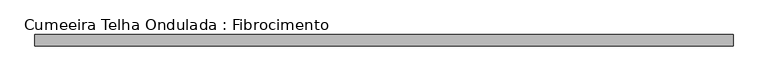
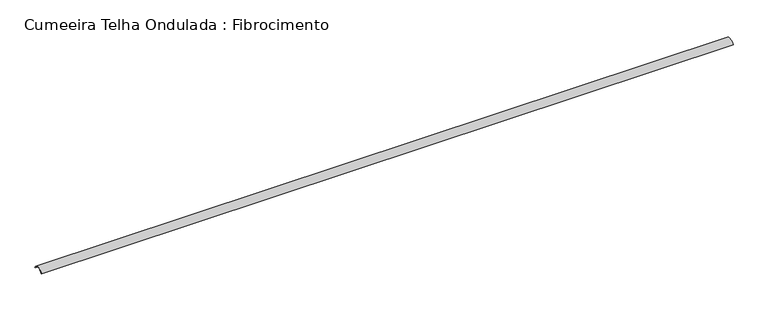
"""IFC4 building model written with IfcOpenShell, lengths in millimetres: beam geometry, Cumeeira Telha Ondulada : Fibrocimento."""

import ifcopenshell
import ifcopenshell.guid

model = None  # the IFC model being written
_history = None  # IfcOwnerHistory: only IFC2X3 demands one
_inside = {}  # id of a spatial element -> (the spatial element, [elements in it])
_under = {}  # id of a project, library or spatial element -> (it, [spatial elements below it])
_declared = {}  # id of a project -> (the project, [libraries it declares])
_typed = {}  # id of a type object -> (the type object, [elements of that type])
_made_of = {}  # id of a material, layer set ... -> (it, [elements and type objects made of it])


def new_model(schema):
    """Start an empty IFC model of exactly this schema.

    Asked for "IFC4X3", IfcOpenShell would pick the latest addendum, in which some entities
    have other attributes; the version numbers below select the first issue.
    IFC2X3 requires an IfcOwnerHistory on every rooted entity: one is made here for all.
    """
    global model, _history
    if schema == "IFC4X3":
        model = ifcopenshell.file(schema_version=(4, 3, 0, 0))
    else:
        model = ifcopenshell.file(schema=schema)
    _inside.clear()
    _under.clear()
    _declared.clear()
    _typed.clear()
    _made_of.clear()
    _history = None
    if model.schema == "IFC2X3":
        org = make("IfcOrganization", Name="unknown")
        user = make(
            "IfcPersonAndOrganization",
            ThePerson=make("IfcPerson", FamilyName="unknown"),
            TheOrganization=org,
        )
        app = make(
            "IfcApplication",
            ApplicationDeveloper=org,
            Version="unknown",
            ApplicationFullName="unknown",
            ApplicationIdentifier="unknown",
        )
        _history = make(
            "IfcOwnerHistory",
            OwningUser=user,
            OwningApplication=app,
            ChangeAction="ADDED",
            CreationDate=0,
        )
    return model


def make(cls, **values):
    """One entity of the class cls with the attributes given. An attribute that is None is left unset."""
    return model.create_entity(
        cls, **{name: value for name, value in values.items() if value is not None}
    )


def rooted(cls, **values):
    """An entity with a GlobalId (a new one), such as an element, a storey or a relation."""
    return make(cls, GlobalId=ifcopenshell.guid.new(), OwnerHistory=_history, **values)


def si_unit(unit_type, name, prefix=None):
    """IfcSIUnit, for example si_unit("LENGTHUNIT", "METRE", prefix="MILLI")."""
    return make("IfcSIUnit", UnitType=unit_type, Prefix=prefix, Name=name)


def assignment(units):
    """IfcUnitAssignment: the units of a project."""
    return None if units is None else make("IfcUnitAssignment", Units=units)


def point(xyz):
    """IfcCartesianPoint."""
    return None if xyz is None else make("IfcCartesianPoint", Coordinates=xyz)


def direction(xyz):
    """IfcDirection."""
    return None if xyz is None else make("IfcDirection", DirectionRatios=xyz)


def frame(location, z_axis=None, x_axis=None):
    """IfcAxis2Placement3D, a coordinate frame: its origin and axes. An axis left out is left unset."""
    return make(
        "IfcAxis2Placement3D",
        Location=point(location),
        Axis=direction(z_axis),
        RefDirection=direction(x_axis),
    )


def frame_2d(location, x_axis=None):
    """IfcAxis2Placement2D, a coordinate frame in the plane: its origin and x axis."""
    return make(
        "IfcAxis2Placement2D", Location=point(location), RefDirection=direction(x_axis)
    )


def origin():
    """The frame at (0, 0, 0) with its axes left unset."""
    return frame((0.0, 0.0, 0.0))


def place(relative_to, where):
    """IfcLocalPlacement: puts the frame where relative to a parent placement (None: the world)."""
    return make(
        "IfcLocalPlacement", PlacementRelTo=relative_to, RelativePlacement=where
    )


def context(
    kind, dimensions, precision=None, world=None, true_north=None, identifier=None
):
    """IfcGeometricRepresentationContext, for example the 3D "Model" context."""
    return make(
        "IfcGeometricRepresentationContext",
        ContextIdentifier=identifier,
        ContextType=kind,
        CoordinateSpaceDimension=dimensions,
        Precision=precision,
        WorldCoordinateSystem=world,
        TrueNorth=true_north,
    )


def project(units=None, contexts=None):
    """IfcProject with its units and contexts."""
    return rooted(
        "IfcProject",
        Name="project",
        RepresentationContexts=contexts,
        UnitsInContext=assignment(units),
    )


def spatial(cls, under=None, at=None, **own):
    """A site, building, storey or space (cls), placed at a placement, below another one or the project."""
    s = rooted(cls, ObjectPlacement=at, **own)
    if under is not None:
        _under.setdefault(under.id(), (under, []))[1].append(s)
    return s


def polyline(points):
    """IfcPolyline through the points."""
    return make("IfcPolyline", Points=[point(p) for p in points])


def circle_curve(where, radius):
    """IfcCircle in the frame where."""
    return make("IfcCircle", Position=where, Radius=radius)


def trimmed(basis, trim1, trim2, sense, master):
    """IfcTrimmedCurve: the piece of a basis curve between two trims."""
    return make(
        "IfcTrimmedCurve",
        BasisCurve=basis,
        Trim1=trim1,
        Trim2=trim2,
        SenseAgreement=sense,
        MasterRepresentation=master,
    )


def segment(curve, same_sense, transition):
    """IfcCompositeCurveSegment."""
    return make(
        "IfcCompositeCurveSegment",
        Transition=transition,
        SameSense=same_sense,
        ParentCurve=curve,
    )


def composite_curve(segments, self_intersect=None):
    """IfcCompositeCurve: segments joined end to end."""
    return make("IfcCompositeCurve", Segments=segments, SelfIntersect=self_intersect)


def outline(outer, holes=None, kind="AREA"):
    """IfcArbitraryClosedProfileDef: a profile drawn as a closed curve; with holes, ...WithVoids."""
    if holes is None:
        return make("IfcArbitraryClosedProfileDef", ProfileType=kind, OuterCurve=outer)
    return make(
        "IfcArbitraryProfileDefWithVoids",
        ProfileType=kind,
        OuterCurve=outer,
        InnerCurves=holes,
    )


def extrude(swept, where, along, depth):
    """IfcExtrudedAreaSolid: the profile swept, set in the frame where, extruded along a direction by depth."""
    return make(
        "IfcExtrudedAreaSolid",
        SweptArea=swept,
        Position=where,
        ExtrudedDirection=direction(along),
        Depth=depth,
    )


def shape(context_of_items, identifier, shape_type, items):
    """IfcShapeRepresentation: the items that make up one representation, for example the "Body"."""
    return make(
        "IfcShapeRepresentation",
        ContextOfItems=context_of_items,
        RepresentationIdentifier=identifier,
        RepresentationType=shape_type,
        Items=items,
    )


def source(mapping_origin, context_of_items, identifier, shape_type, items):
    """IfcRepresentationMap: a shape defined once, which mapped items show again and again."""
    return make(
        "IfcRepresentationMap",
        MappingOrigin=mapping_origin,
        MappedRepresentation=shape(context_of_items, identifier, shape_type, items),
    )


def transform(
    local_origin,
    x_axis=None,
    y_axis=None,
    z_axis=None,
    scale=None,
    scale2=None,
    scale3=None,
    uniform=True,
):
    """IfcCartesianTransformationOperator3D, or its non-uniform kind. x_axis, y_axis, z_axis: its Axis1, 2, 3."""
    if uniform:
        return make(
            "IfcCartesianTransformationOperator3D",
            Axis1=direction(x_axis),
            Axis2=direction(y_axis),
            LocalOrigin=point(local_origin),
            Scale=scale,
            Axis3=direction(z_axis),
        )
    return make(
        "IfcCartesianTransformationOperator3DnonUniform",
        Axis1=direction(x_axis),
        Axis2=direction(y_axis),
        LocalOrigin=point(local_origin),
        Scale=scale,
        Axis3=direction(z_axis),
        Scale2=scale2,
        Scale3=scale3,
    )


def mapped(mapping_source, mapping_target):
    """IfcMappedItem: shows the shape of a source again, moved by a transform."""
    return make(
        "IfcMappedItem", MappingSource=mapping_source, MappingTarget=mapping_target
    )


def made_of(thing, what):
    """Note that an element or type object is made of a material, layer set ...; save() writes the relation."""
    if what is not None:
        _made_of.setdefault(what.id(), (what, []))[1].append(thing)
    return thing


def element(
    cls,
    number,
    at=None,
    inside=None,
    cuts=None,
    type_object=None,
    material=None,
    context=None,
    identifier="Body",
    shape_type=None,
    held_by="IfcProductDefinitionShape",
    body=None,
    shapes=None,
    **own,
):
    """One element of the class cls, such as IfcWall. Its Tag is "e" and its number.

    at: its placement. inside: the storey or other place that contains it. cuts: it is an
    opening in that element (IfcRelVoidsElement). A single representation is given by context,
    identifier, shape_type and body (its items); several are given by shapes. held_by: the class
    of the entity that holds the representations. save() writes the other relations.
    """
    e = rooted(cls, Tag="e%d" % number, ObjectPlacement=at, **own)
    if body is not None:
        shapes = [shape(context, identifier, shape_type, body)]
    if shapes is not None:
        e.Representation = make(held_by, Representations=shapes)
    if inside is not None:
        _inside.setdefault(inside.id(), (inside, []))[1].append(e)
    if cuts is not None:
        rooted(
            "IfcRelVoidsElement", RelatingBuildingElement=cuts, RelatedOpeningElement=e
        )
    if type_object is not None:
        _typed.setdefault(type_object.id(), (type_object, []))[1].append(e)
    return made_of(e, material)


def aggregate(whole, parts):
    """IfcRelAggregates: a whole, such as a stair, and the parts it consists of."""
    return rooted("IfcRelAggregates", RelatingObject=whole, RelatedObjects=parts)


def save(model, path):
    """Write the relations noted so far, then the file.

    IfcRelAggregates (storeys below a building ...), IfcRelContainedInSpatialStructure (elements
    in a storey), IfcRelDefinesByType, IfcRelAssociatesMaterial and IfcRelDeclares: one each for
    every whole, place, type object, material and project.
    """
    for whole, parts in _under.values():
        aggregate(whole, parts)
    for where, things in _inside.values():
        rooted(
            "IfcRelContainedInSpatialStructure",
            RelatedElements=things,
            RelatingStructure=where,
        )
    for kind, things in _typed.values():
        rooted("IfcRelDefinesByType", RelatedObjects=things, RelatingType=kind)
    for what, things in _made_of.values():
        rooted("IfcRelAssociatesMaterial", RelatedObjects=things, RelatingMaterial=what)
    for by, libraries in _declared.values():
        rooted("IfcRelDeclares", RelatingContext=by, RelatedDefinitions=libraries)
    model.write(path)


def cumeeira_telha_ondulada_fibrocimento_28917381(model_context):
    return source(origin(), model_context, "Body", "SweptSolid", [
        extrude(outline(composite_curve([segment(polyline([(58.3970135, 42.4437972), (53.9055884, 40.2467307)]), True, "CONTINUOUS"), segment(trimmed(circle_curve(frame_2d((-1.6029865, 13.0936483)), 61.7939461), [point((53.9055884, 40.2467307))], [point((-57.1115615, 40.2467307))], True, "CARTESIAN"), True, "CONTINUOUS"), segment(polyline([(-57.1115615, 40.2467307), (-61.6029865, 42.4437972)]), True, "CONTINUOUS"), segment(trimmed(circle_curve(frame_2d((-1.6029865, 13.0936483)), 66.7939461), [point((-61.6029865, 42.4437972))], [point((58.3970135, 42.4437972))], False, "CARTESIAN"), True, "CONTINUOUS")], self_intersect=False)), frame((-3626.5, 0.0, 0.0), z_axis=(1.0, 0.0, 0.0), x_axis=(0.0, 1.0, 0.0)), (0.0, 0.0, 1.0), 7253.0),
    ])


if __name__ == "__main__":
    model = new_model("IFC4")
    model_context = context("Model", 3, world=origin())
    ifc_project = project(units=[si_unit("LENGTHUNIT", "METRE", prefix="MILLI")], contexts=[model_context])
    site = spatial("IfcSite", under=ifc_project)
    building = spatial("IfcBuilding", under=site)
    placement = place(None, origin())
    cumeeira_telha_ondulada_fibrocimento_shape = cumeeira_telha_ondulada_fibrocimento_28917381(model_context)
    element("IfcBeam", 1, ObjectType="Cumeeira Telha Ondulada : Fibrocimento", at=placement, inside=building, context=model_context, shape_type="MappedRepresentation", body=[
        mapped(cumeeira_telha_ondulada_fibrocimento_shape, transform((0.0, 0.0, 0.0), x_axis=(1.0, 0.0, 0.0), y_axis=(0.0, 1.0, 0.0), z_axis=(0.0, 0.0, 1.0))),
    ])
    save(model, "model.ifc")

# Revit data of these elements
# Type "Cumeeira Telha Ondulada : Fibrocimento"
#   Cost = 5
#   Length [instance default] = 1.524 m
#   b = 0.07 m
#   h = 0.16 m
#   Structural Material = .TELHA DE FIBROCIMENTO
#   Assembly Code = ""
# Element 1 (IfcBeam, "Cumeeira Telha Ondulada : Fibrocimento")
#   Materials on its faces: ".TELHA DE FIBROCIMENTO"
# Materials
#   ".TELHA DE FIBROCIMENTO": class "CC_TELHADO", colour RGB 77 77 76, transparency 0, Description = "TELHA ONDULADA FIBROCIMENTO", Cost = 0
